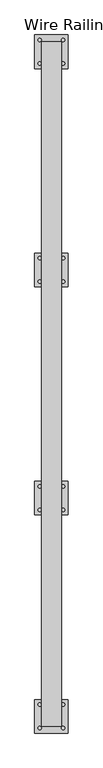
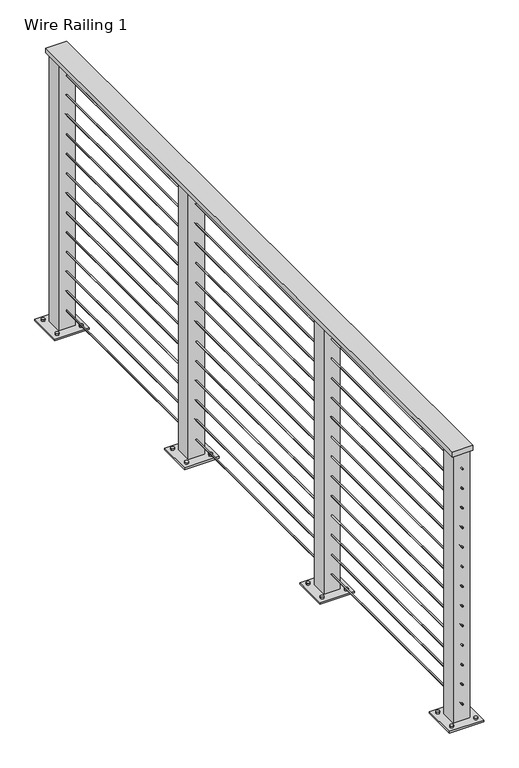
"""IFC4 building model written with IfcOpenShell, lengths in millimetres: railing geometry, Wire Railing 1."""

from ifc_helpers import new_model, si_unit, point, frame, frame_2d, origin, place, context, project, spatial, polyline, circle_curve, trimmed, segment, composite_curve, outline, extrude, source, transform, mapped, element, save


def wire_railing_1_d979133d(model_context):
    return source(origin(), model_context, "Body", "SweptSolid", [
        extrude(outline(polyline([(-134.7929061, -2964.8396465), (-210.9929061, -2964.8396465), (-210.9929061, -374.0396465), (-134.7929061, -374.0396465), (-134.7929061, -2964.8396465)])), frame((0.0, 0.0, 4502.15), z_axis=(0.0, 0.0, 1.0), x_axis=(1.0, 0.0, 0.0)), (0.0, 0.0, 1.0), 19.05),
        extrude(outline(composite_curve([segment(trimmed(circle_curve(frame_2d((4442.61875, -172.8929061)), 2.38125), [point((4442.61875, -175.2741561))], [point((4442.61875, -170.5116561))], False, "CARTESIAN"), True, "CONTINUOUS"), segment(trimmed(circle_curve(frame_2d((4442.61875, -172.8929061)), 2.38125), [point((4442.61875, -170.5116561))], [point((4442.61875, -175.2741561))], False, "CARTESIAN"), True, "CONTINUOUS")], self_intersect=False)), frame((0.0, -2964.8396465, 0.0), z_axis=(0.0, 1.0, 0.0), x_axis=(0.0, 0.0, 1.0)), (0.0, 0.0, 1.0), 2590.8),
        extrude(outline(composite_curve([segment(trimmed(circle_curve(frame_2d((4366.41875, -172.8929061)), 2.38125), [point((4366.41875, -175.2741561))], [point((4366.41875, -170.5116561))], False, "CARTESIAN"), True, "CONTINUOUS"), segment(trimmed(circle_curve(frame_2d((4366.41875, -172.8929061)), 2.38125), [point((4366.41875, -170.5116561))], [point((4366.41875, -175.2741561))], False, "CARTESIAN"), True, "CONTINUOUS")], self_intersect=False)), frame((0.0, -2964.8396465, 0.0), z_axis=(0.0, 1.0, 0.0), x_axis=(0.0, 0.0, 1.0)), (0.0, 0.0, 1.0), 2590.8),
        extrude(outline(composite_curve([segment(trimmed(circle_curve(frame_2d((4290.21875, -172.8929061)), 2.38125), [point((4290.21875, -175.2741561))], [point((4290.21875, -170.5116561))], False, "CARTESIAN"), True, "CONTINUOUS"), segment(trimmed(circle_curve(frame_2d((4290.21875, -172.8929061)), 2.38125), [point((4290.21875, -170.5116561))], [point((4290.21875, -175.2741561))], False, "CARTESIAN"), True, "CONTINUOUS")], self_intersect=False)), frame((0.0, -2964.8396465, 0.0), z_axis=(0.0, 1.0, 0.0), x_axis=(0.0, 0.0, 1.0)), (0.0, 0.0, 1.0), 2590.8),
        extrude(outline(composite_curve([segment(trimmed(circle_curve(frame_2d((4214.01875, -172.8929061)), 2.38125), [point((4214.01875, -175.2741561))], [point((4214.01875, -170.5116561))], False, "CARTESIAN"), True, "CONTINUOUS"), segment(trimmed(circle_curve(frame_2d((4214.01875, -172.8929061)), 2.38125), [point((4214.01875, -170.5116561))], [point((4214.01875, -175.2741561))], False, "CARTESIAN"), True, "CONTINUOUS")], self_intersect=False)), frame((0.0, -2964.8396465, 0.0), z_axis=(0.0, 1.0, 0.0), x_axis=(0.0, 0.0, 1.0)), (0.0, 0.0, 1.0), 2590.8),
        extrude(outline(composite_curve([segment(trimmed(circle_curve(frame_2d((4137.81875, -172.8929061)), 2.38125), [point((4137.81875, -175.2741561))], [point((4137.81875, -170.5116561))], False, "CARTESIAN"), True, "CONTINUOUS"), segment(trimmed(circle_curve(frame_2d((4137.81875, -172.8929061)), 2.38125), [point((4137.81875, -170.5116561))], [point((4137.81875, -175.2741561))], False, "CARTESIAN"), True, "CONTINUOUS")], self_intersect=False)), frame((0.0, -2964.8396465, 0.0), z_axis=(0.0, 1.0, 0.0), x_axis=(0.0, 0.0, 1.0)), (0.0, 0.0, 1.0), 2590.8),
        extrude(outline(composite_curve([segment(trimmed(circle_curve(frame_2d((4061.61875, -172.8929061)), 2.38125), [point((4061.61875, -175.2741561))], [point((4061.61875, -170.5116561))], False, "CARTESIAN"), True, "CONTINUOUS"), segment(trimmed(circle_curve(frame_2d((4061.61875, -172.8929061)), 2.38125), [point((4061.61875, -170.5116561))], [point((4061.61875, -175.2741561))], False, "CARTESIAN"), True, "CONTINUOUS")], self_intersect=False)), frame((0.0, -2964.8396465, 0.0), z_axis=(0.0, 1.0, 0.0), x_axis=(0.0, 0.0, 1.0)), (0.0, 0.0, 1.0), 2590.8),
        extrude(outline(composite_curve([segment(trimmed(circle_curve(frame_2d((3985.41875, -172.8929061)), 2.38125), [point((3985.41875, -175.2741561))], [point((3985.41875, -170.5116561))], False, "CARTESIAN"), True, "CONTINUOUS"), segment(trimmed(circle_curve(frame_2d((3985.41875, -172.8929061)), 2.38125), [point((3985.41875, -170.5116561))], [point((3985.41875, -175.2741561))], False, "CARTESIAN"), True, "CONTINUOUS")], self_intersect=False)), frame((0.0, -2964.8396465, 0.0), z_axis=(0.0, 1.0, 0.0), x_axis=(0.0, 0.0, 1.0)), (0.0, 0.0, 1.0), 2590.8),
        extrude(outline(composite_curve([segment(trimmed(circle_curve(frame_2d((3909.21875, -172.8929061)), 2.38125), [point((3909.21875, -175.2741561))], [point((3909.21875, -170.5116561))], False, "CARTESIAN"), True, "CONTINUOUS"), segment(trimmed(circle_curve(frame_2d((3909.21875, -172.8929061)), 2.38125), [point((3909.21875, -170.5116561))], [point((3909.21875, -175.2741561))], False, "CARTESIAN"), True, "CONTINUOUS")], self_intersect=False)), frame((0.0, -2964.8396465, 0.0), z_axis=(0.0, 1.0, 0.0), x_axis=(0.0, 0.0, 1.0)), (0.0, 0.0, 1.0), 2590.8),
        extrude(outline(composite_curve([segment(trimmed(circle_curve(frame_2d((3833.01875, -172.8929061)), 2.38125), [point((3833.01875, -175.2741561))], [point((3833.01875, -170.5116561))], False, "CARTESIAN"), True, "CONTINUOUS"), segment(trimmed(circle_curve(frame_2d((3833.01875, -172.8929061)), 2.38125), [point((3833.01875, -170.5116561))], [point((3833.01875, -175.2741561))], False, "CARTESIAN"), True, "CONTINUOUS")], self_intersect=False)), frame((0.0, -2964.8396465, 0.0), z_axis=(0.0, 1.0, 0.0), x_axis=(0.0, 0.0, 1.0)), (0.0, 0.0, 1.0), 2590.8),
        extrude(outline(composite_curve([segment(trimmed(circle_curve(frame_2d((3756.81875, -172.8929061)), 2.38125), [point((3756.81875, -175.2741561))], [point((3756.81875, -170.5116561))], False, "CARTESIAN"), True, "CONTINUOUS"), segment(trimmed(circle_curve(frame_2d((3756.81875, -172.8929061)), 2.38125), [point((3756.81875, -170.5116561))], [point((3756.81875, -175.2741561))], False, "CARTESIAN"), True, "CONTINUOUS")], self_intersect=False)), frame((0.0, -2964.8396465, 0.0), z_axis=(0.0, 1.0, 0.0), x_axis=(0.0, 0.0, 1.0)), (0.0, 0.0, 1.0), 2590.8),
        extrude(outline(composite_curve([segment(trimmed(circle_curve(frame_2d((3680.61875, -172.8929061)), 2.38125), [point((3680.61875, -175.2741561))], [point((3680.61875, -170.5116561))], False, "CARTESIAN"), True, "CONTINUOUS"), segment(trimmed(circle_curve(frame_2d((3680.61875, -172.8929061)), 2.38125), [point((3680.61875, -170.5116561))], [point((3680.61875, -175.2741561))], False, "CARTESIAN"), True, "CONTINUOUS")], self_intersect=False)), frame((0.0, -2964.8396465, 0.0), z_axis=(0.0, 1.0, 0.0), x_axis=(0.0, 0.0, 1.0)), (0.0, 0.0, 1.0), 2590.8),
        extrude(outline(composite_curve([segment(trimmed(circle_curve(frame_2d((3604.41875, -172.8929061)), 2.38125), [point((3604.41875, -175.2741561))], [point((3604.41875, -170.5116561))], False, "CARTESIAN"), True, "CONTINUOUS"), segment(trimmed(circle_curve(frame_2d((3604.41875, -172.8929061)), 2.38125), [point((3604.41875, -170.5116561))], [point((3604.41875, -175.2741561))], False, "CARTESIAN"), True, "CONTINUOUS")], self_intersect=False)), frame((0.0, -2964.8396465, 0.0), z_axis=(0.0, 1.0, 0.0), x_axis=(0.0, 0.0, 1.0)), (0.0, 0.0, 1.0), 2590.8),
        extrude(outline(composite_curve([segment(trimmed(circle_curve(frame_2d((3528.21875, -172.8929061)), 2.38125), [point((3528.21875, -175.2741561))], [point((3528.21875, -170.5116561))], False, "CARTESIAN"), True, "CONTINUOUS"), segment(trimmed(circle_curve(frame_2d((3528.21875, -172.8929061)), 2.38125), [point((3528.21875, -170.5116561))], [point((3528.21875, -175.2741561))], False, "CARTESIAN"), True, "CONTINUOUS")], self_intersect=False)), frame((0.0, -2964.8396465, 0.0), z_axis=(0.0, 1.0, 0.0), x_axis=(0.0, 0.0, 1.0)), (0.0, 0.0, 1.0), 2590.8),
        extrude(outline(composite_curve([segment(trimmed(circle_curve(frame_2d((-128.4429061, -1282.0896465)), 6.35), [point((-122.0929061, -1282.0896465))], [point((-134.7929061, -1282.0896465))], False, "CARTESIAN"), True, "CONTINUOUS"), segment(trimmed(circle_curve(frame_2d((-128.4429061, -1282.0896465)), 6.35), [point((-134.7929061, -1282.0896465))], [point((-122.0929061, -1282.0896465))], False, "CARTESIAN"), True, "CONTINUOUS")], self_intersect=False)), frame((0.0, 0.0, 3454.4), z_axis=(0.0, 0.0, 1.0), x_axis=(1.0, 0.0, 0.0)), (0.0, 0.0, 1.0), 12.7),
        extrude(outline(composite_curve([segment(trimmed(circle_curve(frame_2d((-217.3429061, -1282.0896465)), 6.35), [point((-210.9929061, -1282.0896465))], [point((-223.6929061, -1282.0896465))], False, "CARTESIAN"), True, "CONTINUOUS"), segment(trimmed(circle_curve(frame_2d((-217.3429061, -1282.0896465)), 6.35), [point((-223.6929061, -1282.0896465))], [point((-210.9929061, -1282.0896465))], False, "CARTESIAN"), True, "CONTINUOUS")], self_intersect=False)), frame((0.0, 0.0, 3454.4), z_axis=(0.0, 0.0, 1.0), x_axis=(1.0, 0.0, 0.0)), (0.0, 0.0, 1.0), 12.7),
        extrude(outline(composite_curve([segment(trimmed(circle_curve(frame_2d((-128.4429061, -1193.1896465)), 6.35), [point((-122.0929061, -1193.1896465))], [point((-134.7929061, -1193.1896465))], False, "CARTESIAN"), True, "CONTINUOUS"), segment(trimmed(circle_curve(frame_2d((-128.4429061, -1193.1896465)), 6.35), [point((-134.7929061, -1193.1896465))], [point((-122.0929061, -1193.1896465))], False, "CARTESIAN"), True, "CONTINUOUS")], self_intersect=False)), frame((0.0, 0.0, 3454.4), z_axis=(0.0, 0.0, 1.0), x_axis=(1.0, 0.0, 0.0)), (0.0, 0.0, 1.0), 12.7),
        extrude(outline(composite_curve([segment(trimmed(circle_curve(frame_2d((-217.3429061, -1193.1896465)), 6.35), [point((-210.9929061, -1193.1896465))], [point((-223.6929061, -1193.1896465))], False, "CARTESIAN"), True, "CONTINUOUS"), segment(trimmed(circle_curve(frame_2d((-217.3429061, -1193.1896465)), 6.35), [point((-223.6929061, -1193.1896465))], [point((-210.9929061, -1193.1896465))], False, "CARTESIAN"), True, "CONTINUOUS")], self_intersect=False)), frame((0.0, 0.0, 3454.4), z_axis=(0.0, 0.0, 1.0), x_axis=(1.0, 0.0, 0.0)), (0.0, 0.0, 1.0), 12.7),
        extrude(outline(polyline([(-236.3929061, -1301.1396465), (-236.3929061, -1174.1396465), (-109.3929061, -1174.1396465), (-109.3929061, -1301.1396465), (-236.3929061, -1301.1396465)])), frame((0.0, 0.0, 3454.4), z_axis=(0.0, 0.0, 1.0), x_axis=(1.0, 0.0, 0.0)), (0.0, 0.0, 1.0), 6.35),
        extrude(outline(polyline([(-203.0554061, -1267.8021465), (-203.0554061, -1207.4771465), (-142.7304061, -1207.4771465), (-142.7304061, -1267.8021465), (-203.0554061, -1267.8021465)]), holes=[polyline([(-196.7054061, -1261.4521465), (-149.0804061, -1261.4521465), (-149.0804061, -1213.8271465), (-196.7054061, -1213.8271465), (-196.7054061, -1261.4521465)])]), frame((0.0, 0.0, 3454.4), z_axis=(0.0, 0.0, 1.0), x_axis=(1.0, 0.0, 0.0)), (0.0, 0.0, 1.0), 1047.75),
        extrude(outline(composite_curve([segment(trimmed(circle_curve(frame_2d((-128.4429061, -2145.6896465)), 6.35), [point((-122.0929061, -2145.6896465))], [point((-134.7929061, -2145.6896465))], False, "CARTESIAN"), True, "CONTINUOUS"), segment(trimmed(circle_curve(frame_2d((-128.4429061, -2145.6896465)), 6.35), [point((-134.7929061, -2145.6896465))], [point((-122.0929061, -2145.6896465))], False, "CARTESIAN"), True, "CONTINUOUS")], self_intersect=False)), frame((0.0, 0.0, 3454.4), z_axis=(0.0, 0.0, 1.0), x_axis=(1.0, 0.0, 0.0)), (0.0, 0.0, 1.0), 12.7),
        extrude(outline(composite_curve([segment(trimmed(circle_curve(frame_2d((-217.3429061, -2145.6896465)), 6.35), [point((-210.9929061, -2145.6896465))], [point((-223.6929061, -2145.6896465))], False, "CARTESIAN"), True, "CONTINUOUS"), segment(trimmed(circle_curve(frame_2d((-217.3429061, -2145.6896465)), 6.35), [point((-223.6929061, -2145.6896465))], [point((-210.9929061, -2145.6896465))], False, "CARTESIAN"), True, "CONTINUOUS")], self_intersect=False)), frame((0.0, 0.0, 3454.4), z_axis=(0.0, 0.0, 1.0), x_axis=(1.0, 0.0, 0.0)), (0.0, 0.0, 1.0), 12.7),
        extrude(outline(composite_curve([segment(trimmed(circle_curve(frame_2d((-128.4429061, -2056.7896465)), 6.35), [point((-122.0929061, -2056.7896465))], [point((-134.7929061, -2056.7896465))], False, "CARTESIAN"), True, "CONTINUOUS"), segment(trimmed(circle_curve(frame_2d((-128.4429061, -2056.7896465)), 6.35), [point((-134.7929061, -2056.7896465))], [point((-122.0929061, -2056.7896465))], False, "CARTESIAN"), True, "CONTINUOUS")], self_intersect=False)), frame((0.0, 0.0, 3454.4), z_axis=(0.0, 0.0, 1.0), x_axis=(1.0, 0.0, 0.0)), (0.0, 0.0, 1.0), 12.7),
        extrude(outline(composite_curve([segment(trimmed(circle_curve(frame_2d((-217.3429061, -2056.7896465)), 6.35), [point((-210.9929061, -2056.7896465))], [point((-223.6929061, -2056.7896465))], False, "CARTESIAN"), True, "CONTINUOUS"), segment(trimmed(circle_curve(frame_2d((-217.3429061, -2056.7896465)), 6.35), [point((-223.6929061, -2056.7896465))], [point((-210.9929061, -2056.7896465))], False, "CARTESIAN"), True, "CONTINUOUS")], self_intersect=False)), frame((0.0, 0.0, 3454.4), z_axis=(0.0, 0.0, 1.0), x_axis=(1.0, 0.0, 0.0)), (0.0, 0.0, 1.0), 12.7),
        extrude(outline(polyline([(-236.3929061, -2164.7396465), (-236.3929061, -2037.7396465), (-109.3929061, -2037.7396465), (-109.3929061, -2164.7396465), (-236.3929061, -2164.7396465)])), frame((0.0, 0.0, 3454.4), z_axis=(0.0, 0.0, 1.0), x_axis=(1.0, 0.0, 0.0)), (0.0, 0.0, 1.0), 6.35),
        extrude(outline(polyline([(-203.0554061, -2131.4021465), (-203.0554061, -2071.0771465), (-142.7304061, -2071.0771465), (-142.7304061, -2131.4021465), (-203.0554061, -2131.4021465)]), holes=[polyline([(-196.7054061, -2125.0521465), (-149.0804061, -2125.0521465), (-149.0804061, -2077.4271465), (-196.7054061, -2077.4271465), (-196.7054061, -2125.0521465)])]), frame((0.0, 0.0, 3454.4), z_axis=(0.0, 0.0, 1.0), x_axis=(1.0, 0.0, 0.0)), (0.0, 0.0, 1.0), 1047.75),
        extrude(outline(composite_curve([segment(trimmed(circle_curve(frame_2d((-128.4429061, -456.5896465)), 6.35), [point((-122.0929061, -456.5896465))], [point((-134.7929061, -456.5896465))], False, "CARTESIAN"), True, "CONTINUOUS"), segment(trimmed(circle_curve(frame_2d((-128.4429061, -456.5896465)), 6.35), [point((-134.7929061, -456.5896465))], [point((-122.0929061, -456.5896465))], False, "CARTESIAN"), True, "CONTINUOUS")], self_intersect=False)), frame((0.0, 0.0, 3454.4), z_axis=(0.0, 0.0, 1.0), x_axis=(1.0, 0.0, 0.0)), (0.0, 0.0, 1.0), 12.7),
        extrude(outline(composite_curve([segment(trimmed(circle_curve(frame_2d((-217.3429061, -456.5896465)), 6.35), [point((-210.9929061, -456.5896465))], [point((-223.6929061, -456.5896465))], False, "CARTESIAN"), True, "CONTINUOUS"), segment(trimmed(circle_curve(frame_2d((-217.3429061, -456.5896465)), 6.35), [point((-223.6929061, -456.5896465))], [point((-210.9929061, -456.5896465))], False, "CARTESIAN"), True, "CONTINUOUS")], self_intersect=False)), frame((0.0, 0.0, 3454.4), z_axis=(0.0, 0.0, 1.0), x_axis=(1.0, 0.0, 0.0)), (0.0, 0.0, 1.0), 12.7),
        extrude(outline(composite_curve([segment(trimmed(circle_curve(frame_2d((-128.4429061, -367.6896465)), 6.35), [point((-122.0929061, -367.6896465))], [point((-134.7929061, -367.6896465))], False, "CARTESIAN"), True, "CONTINUOUS"), segment(trimmed(circle_curve(frame_2d((-128.4429061, -367.6896465)), 6.35), [point((-134.7929061, -367.6896465))], [point((-122.0929061, -367.6896465))], False, "CARTESIAN"), True, "CONTINUOUS")], self_intersect=False)), frame((0.0, 0.0, 3454.4), z_axis=(0.0, 0.0, 1.0), x_axis=(1.0, 0.0, 0.0)), (0.0, 0.0, 1.0), 12.7),
        extrude(outline(composite_curve([segment(trimmed(circle_curve(frame_2d((-217.3429061, -367.6896465)), 6.35), [point((-210.9929061, -367.6896465))], [point((-223.6929061, -367.6896465))], False, "CARTESIAN"), True, "CONTINUOUS"), segment(trimmed(circle_curve(frame_2d((-217.3429061, -367.6896465)), 6.35), [point((-223.6929061, -367.6896465))], [point((-210.9929061, -367.6896465))], False, "CARTESIAN"), True, "CONTINUOUS")], self_intersect=False)), frame((0.0, 0.0, 3454.4), z_axis=(0.0, 0.0, 1.0), x_axis=(1.0, 0.0, 0.0)), (0.0, 0.0, 1.0), 12.7),
        extrude(outline(polyline([(-236.3929061, -475.6396465), (-236.3929061, -348.6396465), (-109.3929061, -348.6396465), (-109.3929061, -475.6396465), (-236.3929061, -475.6396465)])), frame((0.0, 0.0, 3454.4), z_axis=(0.0, 0.0, 1.0), x_axis=(1.0, 0.0, 0.0)), (0.0, 0.0, 1.0), 6.35),
        extrude(outline(polyline([(-203.0554061, -442.3021465), (-203.0554061, -381.9771465), (-142.7304061, -381.9771465), (-142.7304061, -442.3021465), (-203.0554061, -442.3021465)]), holes=[polyline([(-196.7054061, -435.9521465), (-149.0804061, -435.9521465), (-149.0804061, -388.3271465), (-196.7054061, -388.3271465), (-196.7054061, -435.9521465)])]), frame((0.0, 0.0, 3454.4), z_axis=(0.0, 0.0, 1.0), x_axis=(1.0, 0.0, 0.0)), (0.0, 0.0, 1.0), 1047.75),
        extrude(outline(composite_curve([segment(trimmed(circle_curve(frame_2d((-128.4429061, -2971.1896465)), 6.35), [point((-122.0929061, -2971.1896465))], [point((-134.7929061, -2971.1896465))], False, "CARTESIAN"), True, "CONTINUOUS"), segment(trimmed(circle_curve(frame_2d((-128.4429061, -2971.1896465)), 6.35), [point((-134.7929061, -2971.1896465))], [point((-122.0929061, -2971.1896465))], False, "CARTESIAN"), True, "CONTINUOUS")], self_intersect=False)), frame((0.0, 0.0, 3454.4), z_axis=(0.0, 0.0, 1.0), x_axis=(1.0, 0.0, 0.0)), (0.0, 0.0, 1.0), 12.7),
        extrude(outline(composite_curve([segment(trimmed(circle_curve(frame_2d((-217.3429061, -2971.1896465)), 6.35), [point((-210.9929061, -2971.1896465))], [point((-223.6929061, -2971.1896465))], False, "CARTESIAN"), True, "CONTINUOUS"), segment(trimmed(circle_curve(frame_2d((-217.3429061, -2971.1896465)), 6.35), [point((-223.6929061, -2971.1896465))], [point((-210.9929061, -2971.1896465))], False, "CARTESIAN"), True, "CONTINUOUS")], self_intersect=False)), frame((0.0, 0.0, 3454.4), z_axis=(0.0, 0.0, 1.0), x_axis=(1.0, 0.0, 0.0)), (0.0, 0.0, 1.0), 12.7),
        extrude(outline(composite_curve([segment(trimmed(circle_curve(frame_2d((-128.4429061, -2882.2896465)), 6.35), [point((-122.0929061, -2882.2896465))], [point((-134.7929061, -2882.2896465))], False, "CARTESIAN"), True, "CONTINUOUS"), segment(trimmed(circle_curve(frame_2d((-128.4429061, -2882.2896465)), 6.35), [point((-134.7929061, -2882.2896465))], [point((-122.0929061, -2882.2896465))], False, "CARTESIAN"), True, "CONTINUOUS")], self_intersect=False)), frame((0.0, 0.0, 3454.4), z_axis=(0.0, 0.0, 1.0), x_axis=(1.0, 0.0, 0.0)), (0.0, 0.0, 1.0), 12.7),
        extrude(outline(composite_curve([segment(trimmed(circle_curve(frame_2d((-217.3429061, -2882.2896465)), 6.35), [point((-210.9929061, -2882.2896465))], [point((-223.6929061, -2882.2896465))], False, "CARTESIAN"), True, "CONTINUOUS"), segment(trimmed(circle_curve(frame_2d((-217.3429061, -2882.2896465)), 6.35), [point((-223.6929061, -2882.2896465))], [point((-210.9929061, -2882.2896465))], False, "CARTESIAN"), True, "CONTINUOUS")], self_intersect=False)), frame((0.0, 0.0, 3454.4), z_axis=(0.0, 0.0, 1.0), x_axis=(1.0, 0.0, 0.0)), (0.0, 0.0, 1.0), 12.7),
        extrude(outline(polyline([(-236.3929061, -2990.2396465), (-236.3929061, -2863.2396465), (-109.3929061, -2863.2396465), (-109.3929061, -2990.2396465), (-236.3929061, -2990.2396465)])), frame((0.0, 0.0, 3454.4), z_axis=(0.0, 0.0, 1.0), x_axis=(1.0, 0.0, 0.0)), (0.0, 0.0, 1.0), 6.35),
        extrude(outline(polyline([(-203.0554061, -2956.9021465), (-203.0554061, -2896.5771465), (-142.7304061, -2896.5771465), (-142.7304061, -2956.9021465), (-203.0554061, -2956.9021465)]), holes=[polyline([(-196.7054061, -2950.5521465), (-149.0804061, -2950.5521465), (-149.0804061, -2902.9271465), (-196.7054061, -2902.9271465), (-196.7054061, -2950.5521465)])]), frame((0.0, 0.0, 3454.4), z_axis=(0.0, 0.0, 1.0), x_axis=(1.0, 0.0, 0.0)), (0.0, 0.0, 1.0), 1047.75),
    ])


if __name__ == "__main__":
    model = new_model("IFC4")
    model_context = context("Model", 3, world=origin())
    ifc_project = project(units=[si_unit("LENGTHUNIT", "METRE", prefix="MILLI")], contexts=[model_context])
    site = spatial("IfcSite", under=ifc_project)
    building = spatial("IfcBuilding", under=site)
    placement = place(None, origin())
    wire_railing_1_shape = wire_railing_1_d979133d(model_context)
    element("IfcRailing", 1, ObjectType="Wire Railing 1", at=placement, inside=building, context=model_context, shape_type="MappedRepresentation", body=[
        mapped(wire_railing_1_shape, transform((0.0, 0.0, 0.0), x_axis=(1.0, 0.0, 0.0), y_axis=(0.0, 1.0, 0.0), z_axis=(0.0, 0.0, 1.0))),
    ])
    save(model, "model.ifc")

# Revit data of these elements
# Element 1 (IfcRailing, "Wire Railing 1")
#   Materials on its faces: "Metal - Kawneer - Aluminum"
# Materials
#   "Metal - Kawneer - Aluminum": class "Metal", colour RGB 244 244 244, transparency 0, Manufacturer = "Kawneer", URL = "http://www.kawneer.com/kawneer/north_america/en/home.asp", Cost = 0
